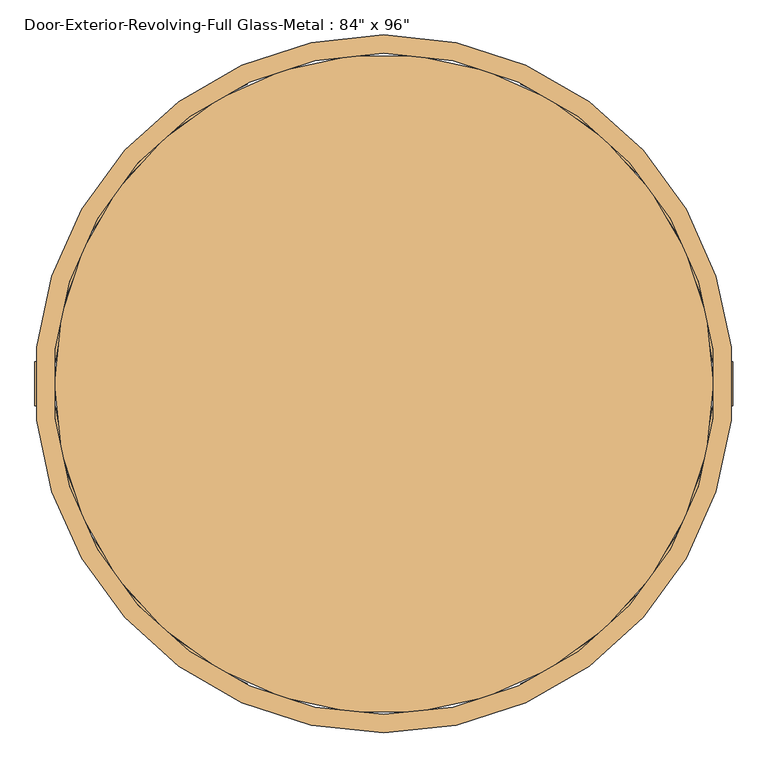
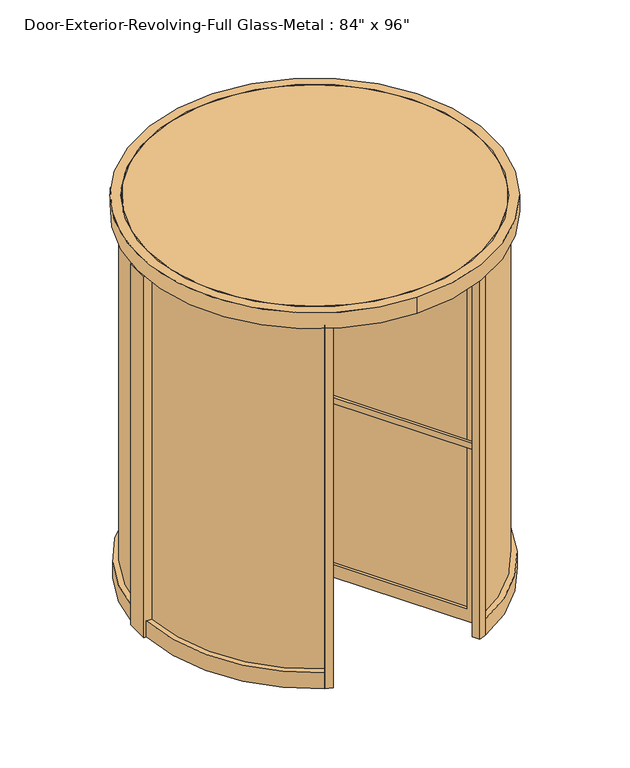
"""IFC4 building model written with IfcOpenShell, lengths in millimetres: door geometry."""

from ifc_helpers import new_model, si_unit, point, frame, frame_2d, origin, origin_with_axes, origin_2d, place, context, project, spatial, polyline, circle_curve, trimmed, segment, composite_curve, outline, extrude, source, transform, mapped, element, save
from ifc_brep_helpers import plane_surface, revolved_surface, advanced_brep


def door_2695eedf(model_context):
    return source(origin(), model_context, "Body", "SolidModel", [
        advanced_brep(
        [(481.9772161, -872.9090263, 25.4), (481.9772161, -872.9090263, 2282.825), (26.9196881, -84.7262674, 2282.825), (26.9196881, -84.7262674, 25.4), (29.5397161, -89.2642891, 2216.15), (448.6397161, -815.1667825, 2216.15), (448.6397161, -815.1667825, 106.3625), (29.5397161, -89.2642891, 106.3625), (514.9727839, -853.8590263, 2282.825), (514.9727839, -853.8590263, 25.4), (59.9152559, -65.6762674, 25.4), (59.9152559, -65.6762674, 2282.825), (62.5352839, -70.2142891, 2216.15), (62.5352839, -70.2142891, 106.3625), (481.6352839, -796.1167825, 106.3625), (481.6352839, -796.1167825, 2216.15), (44.45, -76.9896584, 2282.825), (44.45, -76.9896584, 25.4)],
        [
            (0, 1),
            (1, 2),
            (2, 3),
            (3, 0),
            (4, 5),
            (5, 6),
            (6, 7),
            (7, 4),
            (8, 9),
            (9, 10),
            (10, 11),
            (11, 8),
            (12, 13),
            (13, 14),
            (14, 15),
            (15, 12),
            (1, 8),
            (11, 16, circle_curve(frame((0.0, 0.0, 2282.825), z_axis=(0.0, 0.0, -1.0), x_axis=(0.4999999999999996, -0.8660254037844389, 0.0)), 88.9)),
            (16, 2, circle_curve(frame((0.0, 0.0, 2282.825), z_axis=(0.0, 0.0, -1.0), x_axis=(0.4999999999999996, -0.8660254037844389, 0.0)), 88.9)),
            (0, 9),
            (3, 17, circle_curve(frame((0.0, 0.0, 25.4), z_axis=(0.0, 0.0, 1.0), x_axis=(0.4999999999999996, -0.8660254037844389, 0.0)), 88.9)),
            (17, 10, circle_curve(frame((0.0, 0.0, 25.4), z_axis=(0.0, 0.0, 1.0), x_axis=(0.4999999999999996, -0.8660254037844389, 0.0)), 88.9)),
            (7, 13),
            (12, 4),
            (6, 14),
            (5, 15),
            (16, 17),
        ],
        [
            plane_surface(frame((-3.7977839, -31.5220453, 2282.825), z_axis=(-0.8660254037844389, -0.4999999999999996, 0.0), x_axis=(0.0, 0.0, -1.0))),
            plane_surface(frame((29.1977839, -12.4720453, 2282.825), z_axis=(0.8660254037844389, 0.4999999999999996, 0.0), x_axis=(0.0, 0.0, 1.0))),
            plane_surface(frame((481.9772161, -872.9090263, 2282.825), z_axis=(0.0, 0.0, 1.0), x_axis=(0.8660254037844384, 0.5000000000000004, 0.0))),
            plane_surface(frame((481.9772161, -872.9090263, 25.4), z_axis=(0.5000000000000004, -0.8660254037844384, 0.0), x_axis=(0.8660254037844384, 0.5000000000000004, 0.0))),
            plane_surface(frame((-3.7977839, -31.5220453, 25.4), z_axis=(0.0, 0.0, -1.0), x_axis=(0.8660254037844389, 0.49999999999999956, 0.0))),
            plane_surface(frame((29.5397161, -89.2642891, 106.3625), z_axis=(0.4999999999999998, -0.8660254037844388, 0.0), x_axis=(0.8660254037844388, 0.4999999999999998, 0.0))),
            plane_surface(frame((448.6397161, -815.1667825, 106.3625), z_axis=(0.0, 0.0, 1.0), x_axis=(0.8660254037844384, 0.5000000000000004, 0.0))),
            plane_surface(frame((448.6397161, -815.1667825, 2216.15), z_axis=(-0.5000000000000004, 0.8660254037844384, 0.0), x_axis=(0.8660254037844384, 0.5000000000000004, 0.0))),
            plane_surface(frame((29.5397161, -89.2642891, 2216.15), z_axis=(0.0, 0.0, -1.0), x_axis=(0.8660254037844389, 0.49999999999999967, 0.0))),
            revolved_surface(polyline([(44.44999999999997, -76.98965839643662, 2282.825), (44.44999999999997, -76.98965839643662, 25.399999999999977)]), (0.0, 0.0, -344.4385455), (0.0, 0.0, 1.0)),
        ],
        [
            (0, [[1, 2, 3, 4], [5, 6, 7, 8]]),
            (1, [[9, 10, 11, 12], [13, 14, 15, 16]]),
            (2, [[17, -12, 18, 19, -2]]),
            (3, [[-1, 20, -9, -17]]),
            (4, [[-20, -4, 21, 22, -10]]),
            (5, [[-8, 23, -13, 24]]),
            (6, [[-7, 25, -14, -23]]),
            (7, [[-6, 26, -15, -25]]),
            (8, [[-5, -24, -16, -26]]),
            (9, [[27, -21, -3, -19]]),
            (9, [[-27, -18, -11, -22]]),
        ],
    ),
        advanced_brep(
        [(-996.95, -19.05, 2282.825), (-996.95, -19.05, 25.4), (-86.834944, -19.05, 25.4), (-86.834944, -19.05, 2282.825), (-92.075, -19.05, 2216.15), (-92.075, -19.05, 106.3625), (-930.275, -19.05, 106.3625), (-930.275, -19.05, 2216.15), (-996.95, 19.05, 25.4), (-996.95, 19.05, 2282.825), (-86.834944, 19.05, 2282.825), (-86.834944, 19.05, 25.4), (-92.075, 19.05, 2216.15), (-930.275, 19.05, 2216.15), (-930.275, 19.05, 106.3625), (-92.075, 19.05, 106.3625)],
        [
            (0, 1),
            (1, 2),
            (2, 3),
            (3, 0),
            (4, 5),
            (5, 6),
            (6, 7),
            (7, 4),
            (8, 9),
            (9, 10),
            (10, 11),
            (11, 8),
            (12, 13),
            (13, 14),
            (14, 15),
            (15, 12),
            (9, 0),
            (3, 10, circle_curve(frame((0.0, 0.0, 2282.825), z_axis=(0.0, 0.0, -1.0), x_axis=(0.4999999999999996, -0.8660254037844389, 0.0)), 88.9)),
            (8, 1),
            (11, 2, circle_curve(frame((0.0, 0.0, 25.4), z_axis=(0.0, 0.0, 1.0), x_axis=(0.4999999999999996, -0.8660254037844389, 0.0)), 88.9)),
            (4, 12),
            (15, 5),
            (14, 6),
            (13, 7),
        ],
        [
            plane_surface(frame((-996.95, -19.05, 2282.825), z_axis=(0.0, -1.0, 0.0), x_axis=(-1.0, 0.0, 0.0))),
            plane_surface(frame((-996.95, 19.05, 2282.825), z_axis=(0.0, 1.0, 0.0), x_axis=(1.0, 0.0, 0.0))),
            plane_surface(frame((-25.4, -19.05, 2282.825), z_axis=(0.0, 0.0, 1.0), x_axis=(0.0, 1.0, 0.0))),
            plane_surface(frame((-996.95, -19.05, 2282.825), z_axis=(-1.0, 0.0, 0.0), x_axis=(0.0, 1.0, 0.0))),
            plane_surface(frame((-996.95, -19.05, 25.4), z_axis=(0.0, 0.0, -1.0), x_axis=(0.0, 1.0, 0.0))),
            plane_surface(frame((-92.075, -19.05, 2216.15), z_axis=(-1.0, 0.0, 0.0), x_axis=(0.0, 1.0, 0.0))),
            plane_surface(frame((-92.075, -19.05, 106.3625), z_axis=(0.0, 0.0, 1.0), x_axis=(0.0, 1.0, 0.0))),
            plane_surface(frame((-930.275, -19.05, 106.3625), z_axis=(1.0, 0.0, 0.0), x_axis=(0.0, 1.0, 0.0))),
            plane_surface(frame((-930.275, -19.05, 2216.15), z_axis=(0.0, 0.0, -1.0), x_axis=(0.0, 1.0, 0.0))),
            revolved_surface(polyline([(44.44999999999997, -76.98965839643662, 2282.825), (44.44999999999997, -76.98965839643662, 25.399999999999977)]), (0.0, 0.0, -344.4385455), (0.0, 0.0, 1.0)),
        ],
        [
            (0, [[1, 2, 3, 4], [5, 6, 7, 8]]),
            (1, [[9, 10, 11, 12], [13, 14, 15, 16]]),
            (2, [[17, -4, 18, -10]]),
            (3, [[-1, -17, -9, 19]]),
            (4, [[-19, -12, 20, -2]]),
            (5, [[-5, 21, -16, 22]]),
            (6, [[-6, -22, -15, 23]]),
            (7, [[-7, -23, -14, 24]]),
            (8, [[-8, -24, -13, -21]]),
            (9, [[-3, -20, -11, -18]]),
        ],
    ),
        advanced_brep(
        [(514.9727839, 853.8590263, 25.4), (514.9727839, 853.8590263, 2282.825), (59.9152559, 65.6762674, 2282.825), (59.9152559, 65.6762674, 25.4), (62.5352839, 70.2142891, 2216.15), (481.6352839, 796.1167825, 2216.15), (481.6352839, 796.1167825, 106.3625), (62.5352839, 70.2142891, 106.3625), (481.9772161, 872.9090263, 2282.825), (481.9772161, 872.9090263, 25.4), (26.9196881, 84.7262674, 25.4), (26.9196881, 84.7262674, 2282.825), (29.5397161, 89.2642891, 2216.15), (29.5397161, 89.2642891, 106.3625), (448.6397161, 815.1667825, 106.3625), (448.6397161, 815.1667825, 2216.15)],
        [
            (0, 1),
            (1, 2),
            (2, 3),
            (3, 0),
            (4, 5),
            (5, 6),
            (6, 7),
            (7, 4),
            (8, 9),
            (9, 10),
            (10, 11),
            (11, 8),
            (12, 13),
            (13, 14),
            (14, 15),
            (15, 12),
            (1, 8),
            (11, 2, circle_curve(frame((0.0, 0.0, 2282.825), z_axis=(0.0, 0.0, -1.0), x_axis=(0.4999999999999996, -0.8660254037844389, 0.0)), 88.9)),
            (0, 9),
            (3, 10, circle_curve(frame((0.0, 0.0, 25.4), z_axis=(0.0, 0.0, 1.0), x_axis=(0.4999999999999996, -0.8660254037844389, 0.0)), 88.9)),
            (7, 13),
            (12, 4),
            (6, 14),
            (5, 15),
        ],
        [
            plane_surface(frame((29.1977839, 12.4720453, 2282.825), z_axis=(0.866025403784439, -0.4999999999999995, 0.0), x_axis=(0.0, 0.0, -1.0))),
            plane_surface(frame((-3.7977839, 31.5220453, 2282.825), z_axis=(-0.866025403784439, 0.4999999999999995, 0.0), x_axis=(0.0, 0.0, 1.0))),
            plane_surface(frame((514.9727839, 853.8590263, 2282.825), z_axis=(0.0, 0.0, 1.0), x_axis=(-0.8660254037844384, 0.5000000000000004, 0.0))),
            plane_surface(frame((514.9727839, 853.8590263, 25.4), z_axis=(0.5000000000000004, 0.8660254037844384, 0.0), x_axis=(-0.8660254037844384, 0.5000000000000004, 0.0))),
            plane_surface(frame((29.1977839, 12.4720453, 25.4), z_axis=(0.0, 0.0, -1.0), x_axis=(-0.866025403784439, 0.49999999999999944, 0.0))),
            plane_surface(frame((62.5352839, 70.2142891, 106.3625), z_axis=(0.49999999999999956, 0.8660254037844389, 0.0), x_axis=(-0.8660254037844389, 0.49999999999999956, 0.0))),
            plane_surface(frame((481.6352839, 796.1167825, 106.3625), z_axis=(0.0, 0.0, 1.0), x_axis=(-0.8660254037844384, 0.5000000000000004, 0.0))),
            plane_surface(frame((481.6352839, 796.1167825, 2216.15), z_axis=(-0.5000000000000004, -0.8660254037844384, 0.0), x_axis=(-0.8660254037844384, 0.5000000000000004, 0.0))),
            plane_surface(frame((62.5352839, 70.2142891, 2216.15), z_axis=(0.0, 0.0, -1.0), x_axis=(-0.866025403784439, 0.49999999999999944, 0.0))),
            revolved_surface(polyline([(44.44999999999997, -76.98965839643662, 2282.825), (44.44999999999997, -76.98965839643662, 25.399999999999977)]), (0.0, 0.0, -344.4385455), (0.0, 0.0, 1.0)),
        ],
        [
            (0, [[1, 2, 3, 4], [5, 6, 7, 8]]),
            (1, [[9, 10, 11, 12], [13, 14, 15, 16]]),
            (2, [[17, -12, 18, -2]]),
            (3, [[-1, 19, -9, -17]]),
            (4, [[-19, -4, 20, -10]]),
            (5, [[-8, 21, -13, 22]]),
            (6, [[-7, 23, -14, -21]]),
            (7, [[-6, 24, -15, -23]]),
            (8, [[-5, -22, -16, -24]]),
            (9, [[-3, -18, -11, -20]]),
        ],
    ),
        extrude(outline(composite_curve([segment(polyline([(-463.3921907, 900.6009984), (-485.7275667, 942.9715583)]), True, "CONTINUOUS"), segment(trimmed(circle_curve(origin_2d(), 1060.7198635), [point((-485.7275667, 942.9715583))], [point((-443.2078601, 963.6874086))], False, "CARTESIAN"), True, "CONTINUOUS"), segment(polyline([(-443.2078601, 963.6874086), (-420.8795251, 921.2355323)]), True, "CONTINUOUS"), segment(trimmed(circle_curve(origin_2d(), 1012.825), [point((-420.8795251, 921.2355323))], [point((-463.3921907, 900.6009984))], True, "CARTESIAN"), True, "CONTINUOUS")], self_intersect=False)), origin_with_axes(), (0.0, 0.0, 1.0), 2308.225),
        extrude(outline(composite_curve([segment(polyline([(485.8334006, 943.1723269), (463.3921907, 900.6009984)]), True, "CONTINUOUS"), segment(trimmed(circle_curve(origin_2d(), 1012.825), [point((463.3921907, 900.6009984))], [point((420.8795251, 921.2355323))], True, "CARTESIAN"), True, "CONTINUOUS"), segment(polyline([(420.8795251, 921.2355323), (443.3136707, 963.8885416)]), True, "CONTINUOUS"), segment(trimmed(circle_curve(origin_2d(), 1060.9468089), [point((443.3136707, 963.8885416))], [point((485.8334006, 943.1723269))], False, "CARTESIAN"), True, "CONTINUOUS")], self_intersect=False)), origin_with_axes(), (0.0, 0.0, 1.0), 2308.225),
        extrude(outline(composite_curve([segment(trimmed(circle_curve(origin_2d(), 1012.825), [point((-463.3921907, -900.6009984))], [point((-420.8795251, -921.2355323))], True, "CARTESIAN"), True, "CONTINUOUS"), segment(polyline([(-420.8795251, -921.2355323), (-443.2078601, -959.6749591)]), True, "CONTINUOUS"), segment(trimmed(circle_curve(frame_2d((0.0, 231.0126656)), 1270.4999909), [point((-443.2078601, -959.6749591))], [point((-485.7275667, -942.9715583))], False, "CARTESIAN"), True, "CONTINUOUS"), segment(polyline([(-485.7275667, -942.9715583), (-463.3921907, -900.6009984)]), True, "CONTINUOUS")], self_intersect=False)), origin_with_axes(), (0.0, 0.0, 1.0), 2308.225),
        extrude(outline(composite_curve([segment(trimmed(circle_curve(frame_2d((0.0, 231.0127852)), 1270.5001015), [point((485.7275667, -942.9715583))], [point((443.2078689, -959.6749542))], False, "CARTESIAN"), True, "CONTINUOUS"), segment(polyline([(443.2078689, -959.6749542), (420.8795251, -921.2355323)]), True, "CONTINUOUS"), segment(trimmed(circle_curve(origin_2d(), 1012.825), [point((420.8795251, -921.2355323))], [point((463.3921907, -900.6009984))], True, "CARTESIAN"), True, "CONTINUOUS"), segment(polyline([(463.3921907, -900.6009984), (485.7275667, -942.9715583)]), True, "CONTINUOUS")], self_intersect=False)), origin_with_axes(), (0.0, 0.0, 1.0), 2308.225),
        extrude(outline(composite_curve([segment(polyline([(-1018.5303379, 67.46875), (-1024.8907518, 67.46875)]), True, "CONTINUOUS"), segment(trimmed(circle_curve(origin_2d(), 1027.1090913), [point((-1024.8907518, 67.46875))], [point((-470.5714922, 912.9707312))], False, "CARTESIAN"), True, "CONTINUOUS"), segment(polyline([(-470.5714922, 912.9707312), (-467.3807004, 907.4752681)]), True, "CONTINUOUS"), segment(trimmed(circle_curve(origin_2d(), 1020.7625), [point((-467.3807004, 907.4752681))], [point((-1018.5303379, 67.46875))], True, "CARTESIAN"), True, "CONTINUOUS")], self_intersect=False)), frame((0.0, 0.0, 101.6), z_axis=(0.0, 0.0, 1.0), x_axis=(1.0, 0.0, 0.0)), (0.0, 0.0, 1.0), 2206.625),
        extrude(outline(composite_curve([segment(trimmed(circle_curve(origin_2d(), 1020.7625), [point((1018.5303379, 67.46875))], [point((467.3807004, 907.4752681))], True, "CARTESIAN"), True, "CONTINUOUS"), segment(polyline([(467.3807004, 907.4752681), (470.5714922, 912.9707312)]), True, "CONTINUOUS"), segment(trimmed(circle_curve(origin_2d(), 1027.1090913), [point((470.5714922, 912.9707312))], [point((1024.8907518, 67.46875))], False, "CARTESIAN"), True, "CONTINUOUS"), segment(polyline([(1024.8907518, 67.46875), (1018.5303379, 67.46875)]), True, "CONTINUOUS")], self_intersect=False)), frame((0.0, 0.0, 101.6), z_axis=(0.0, 0.0, 1.0), x_axis=(1.0, 0.0, 0.0)), (0.0, 0.0, 1.0), 2206.625),
        extrude(outline(composite_curve([segment(trimmed(circle_curve(origin_2d(), 1020.7625), [point((-1018.5303379, -67.46875))], [point((-467.3807004, -907.4752681))], True, "CARTESIAN"), True, "CONTINUOUS"), segment(polyline([(-467.3807004, -907.4752681), (-470.5714922, -912.9707312)]), True, "CONTINUOUS"), segment(trimmed(circle_curve(origin_2d(), 1027.1090913), [point((-470.5714922, -912.9707312))], [point((-1024.8907518, -67.46875))], False, "CARTESIAN"), True, "CONTINUOUS"), segment(polyline([(-1024.8907518, -67.46875), (-1018.5303379, -67.46875)]), True, "CONTINUOUS")], self_intersect=False)), frame((0.0, 0.0, 101.6), z_axis=(0.0, 0.0, 1.0), x_axis=(1.0, 0.0, 0.0)), (0.0, 0.0, 1.0), 2206.625),
        extrude(outline(composite_curve([segment(polyline([(1018.5303379, -67.46875), (1024.8907518, -67.46875)]), True, "CONTINUOUS"), segment(trimmed(circle_curve(origin_2d(), 1027.1090913), [point((1024.8907518, -67.46875))], [point((470.5714922, -912.9707312))], False, "CARTESIAN"), True, "CONTINUOUS"), segment(polyline([(470.5714922, -912.9707312), (467.3807004, -907.4752681)]), True, "CONTINUOUS"), segment(trimmed(circle_curve(origin_2d(), 1020.7625), [point((467.3807004, -907.4752681))], [point((1018.5303379, -67.46875))], True, "CARTESIAN"), True, "CONTINUOUS")], self_intersect=False)), frame((0.0, 0.0, 101.6), z_axis=(0.0, 0.0, 1.0), x_axis=(1.0, 0.0, 0.0)), (0.0, 0.0, 1.0), 2206.625),
        extrude(outline(composite_curve([segment(trimmed(circle_curve(origin_2d(), 1073.15), [point((0.0, -1073.15))], [point((0.0, 1073.15))], False, "CARTESIAN"), True, "CONTINUOUS"), segment(trimmed(circle_curve(origin_2d(), 1073.15), [point((0.0, 1073.15))], [point((0.0, -1073.15))], False, "CARTESIAN"), True, "CONTINUOUS")], self_intersect=False), holes=[composite_curve([segment(trimmed(circle_curve(origin_2d(), 1016.0), [point((0.0, 1016.0))], [point((0.0, -1016.0))], True, "CARTESIAN"), True, "CONTINUOUS"), segment(trimmed(circle_curve(origin_2d(), 1016.0), [point((0.0, -1016.0))], [point((0.0, 1016.0))], True, "CARTESIAN"), True, "CONTINUOUS")], self_intersect=False)]), frame((0.0, 0.0, 2308.225), z_axis=(0.0, 0.0, 1.0), x_axis=(1.0, 0.0, 0.0)), (0.0, 0.0, 1.0), 101.6),
        extrude(outline(composite_curve([segment(trimmed(circle_curve(origin_2d(), 1012.825), [point((-1012.825, 0.0))], [point((1012.825, 0.0))], False, "CARTESIAN"), True, "CONTINUOUS"), segment(trimmed(circle_curve(origin_2d(), 1012.825), [point((1012.825, 0.0))], [point((-1012.825, 0.0))], False, "CARTESIAN"), True, "CONTINUOUS")], self_intersect=False)), frame((0.0, 0.0, 2308.225), z_axis=(0.0, 0.0, 1.0), x_axis=(1.0, 0.0, 0.0)), (0.0, 0.0, 1.0), 101.6),
        extrude(outline(composite_curve([segment(trimmed(circle_curve(origin_2d(), 88.9), [point((-88.9, 0.0))], [point((88.9, 0.0))], False, "CARTESIAN"), True, "CONTINUOUS"), segment(trimmed(circle_curve(origin_2d(), 88.9), [point((88.9, 0.0))], [point((-88.9, 0.0))], False, "CARTESIAN"), True, "CONTINUOUS")], self_intersect=False)), origin_with_axes(), (0.0, 0.0, 1.0), 2308.225),
        extrude(outline(composite_curve([segment(polyline([(-463.3921907, -900.6009984), (-485.7275667, -942.9715583)]), True, "CONTINUOUS"), segment(trimmed(circle_curve(origin_2d(), 1060.7198635), [point((-485.7275667, -942.9715583))], [point((-1058.571961, -67.46875))], False, "CARTESIAN"), True, "CONTINUOUS"), segment(polyline([(-1058.571961, -67.46875), (-1010.5753057, -67.46875)]), True, "CONTINUOUS"), segment(trimmed(circle_curve(origin_2d(), 1012.825), [point((-1010.5753057, -67.46875))], [point((-463.3921907, -900.6009984))], True, "CARTESIAN"), True, "CONTINUOUS")], self_intersect=False)), origin_with_axes(), (0.0, 0.0, 1.0), 101.6),
        extrude(outline(composite_curve([segment(polyline([(485.7275667, -942.9715583), (463.3921907, -900.6009984)]), True, "CONTINUOUS"), segment(trimmed(circle_curve(origin_2d(), 1012.825), [point((463.3921907, -900.6009984))], [point((1010.5753057, -67.46875))], True, "CARTESIAN"), True, "CONTINUOUS"), segment(polyline([(1010.5753057, -67.46875), (1058.571961, -67.46875)]), True, "CONTINUOUS"), segment(trimmed(circle_curve(origin_2d(), 1060.7198635), [point((1058.571961, -67.46875))], [point((485.7275667, -942.9715583))], False, "CARTESIAN"), True, "CONTINUOUS")], self_intersect=False)), origin_with_axes(), (0.0, 0.0, 1.0), 101.6),
        extrude(outline(composite_curve([segment(polyline([(1058.571961, 67.46875), (1010.5753057, 67.46875)]), True, "CONTINUOUS"), segment(trimmed(circle_curve(origin_2d(), 1012.825), [point((1010.5753057, 67.46875))], [point((463.3921907, 900.6009984))], True, "CARTESIAN"), True, "CONTINUOUS"), segment(polyline([(463.3921907, 900.6009984), (485.7275667, 942.9715583)]), True, "CONTINUOUS"), segment(trimmed(circle_curve(origin_2d(), 1060.7198635), [point((485.7275667, 942.9715583))], [point((1058.571961, 67.46875))], False, "CARTESIAN"), True, "CONTINUOUS")], self_intersect=False)), origin_with_axes(), (0.0, 0.0, 1.0), 101.6),
        extrude(outline(composite_curve([segment(polyline([(-485.7275667, 942.9715583), (-463.3921907, 900.6009984)]), True, "CONTINUOUS"), segment(trimmed(circle_curve(origin_2d(), 1012.825), [point((-463.3921907, 900.6009984))], [point((-1010.5753057, 67.46875))], True, "CARTESIAN"), True, "CONTINUOUS"), segment(polyline([(-1010.5753057, 67.46875), (-1058.571961, 67.46875)]), True, "CONTINUOUS"), segment(trimmed(circle_curve(origin_2d(), 1060.7198635), [point((-1058.571961, 67.46875))], [point((-485.7275667, 942.9715583))], False, "CARTESIAN"), True, "CONTINUOUS")], self_intersect=False)), origin_with_axes(), (0.0, 0.0, 1.0), 101.6),
        extrude(outline(polyline([(-1016.0, 67.46875), (-1016.0, -67.46875), (-1073.15, -67.46875), (-1073.15, 67.46875), (-1016.0, 67.46875)])), origin_with_axes(), (0.0, 0.0, 1.0), 2308.225),
        extrude(outline(polyline([(1073.15, 67.46875), (1073.15, -67.46875), (1016.0, -67.46875), (1016.0, 67.46875), (1073.15, 67.46875)])), origin_with_axes(), (0.0, 0.0, 1.0), 2308.225),
        extrude(outline(polyline([(462.3878693, -807.2292825), (43.2878693, -81.3267891), (48.7871307, -78.1517891), (467.8871307, -804.0542825), (462.3878693, -807.2292825)])), frame((0.0, 0.0, 106.3625), z_axis=(0.0, 0.0, 1.0), x_axis=(1.0, 0.0, 0.0)), (0.0, 0.0, 1.0), 2109.7875),
        extrude(outline(polyline([(467.8871307, 804.0542825), (48.7871307, 78.1517891), (43.2878693, 81.3267891), (462.3878693, 807.2292825), (467.8871307, 804.0542825)])), frame((0.0, 0.0, 106.3625), z_axis=(0.0, 0.0, 1.0), x_axis=(1.0, 0.0, 0.0)), (0.0, 0.0, 1.0), 2109.7875),
        extrude(outline(polyline([(-92.075, -3.175), (-930.275, -3.175), (-930.275, 3.175), (-92.075, 3.175), (-92.075, -3.175)])), frame((0.0, 0.0, 106.3625), z_axis=(0.0, 0.0, 1.0), x_axis=(1.0, 0.0, 0.0)), (0.0, 0.0, 1.0), 2109.7875),
        extrude(outline(composite_curve([segment(polyline([(-996.95, 19.05), (-996.95, 38.1), (-80.3218526, 38.1)]), True, "CONTINUOUS"), segment(trimmed(circle_curve(origin_2d(), 88.9), [point((-80.3218526, 38.1))], [point((-86.834944, 19.05))], True, "CARTESIAN"), True, "CONTINUOUS"), segment(polyline([(-86.834944, 19.05), (-996.95, 19.05)]), True, "CONTINUOUS")], self_intersect=False)), frame((0.0, 0.0, 1149.35), z_axis=(0.0, 0.0, 1.0), x_axis=(1.0, 0.0, 0.0)), (0.0, 0.0, 1.0), 38.1),
        extrude(outline(composite_curve([segment(polyline([(481.9772161, -872.9090263), (465.4794321, -882.4340263), (7.1653584, -88.6107648)]), True, "CONTINUOUS"), segment(trimmed(circle_curve(origin_2d(), 88.9), [point((7.1653584, -88.6107648))], [point((26.9196881, -84.7262674))], True, "CARTESIAN"), True, "CONTINUOUS"), segment(polyline([(26.9196881, -84.7262674), (481.9772161, -872.9090263)]), True, "CONTINUOUS")], self_intersect=False)), frame((0.0, 0.0, 1149.35), z_axis=(0.0, 0.0, 1.0), x_axis=(1.0, 0.0, 0.0)), (0.0, 0.0, 1.0), 38.1),
        extrude(outline(composite_curve([segment(polyline([(514.9727839, 853.8590263), (531.4705679, 844.3340263), (73.1564942, 50.5107648)]), True, "CONTINUOUS"), segment(trimmed(circle_curve(origin_2d(), 88.9), [point((73.1564942, 50.5107648))], [point((59.9152559, 65.6762674))], True, "CARTESIAN"), True, "CONTINUOUS"), segment(polyline([(59.9152559, 65.6762674), (514.9727839, 853.8590263)]), True, "CONTINUOUS")], self_intersect=False)), frame((0.0, 0.0, 1149.35), z_axis=(0.0, 0.0, 1.0), x_axis=(1.0, 0.0, 0.0)), (0.0, 0.0, 1.0), 38.1),
    ])


if __name__ == "__main__":
    model = new_model("IFC4")
    model_context = context("Model", 3, world=origin())
    ifc_project = project(units=[si_unit("LENGTHUNIT", "METRE", prefix="MILLI")], contexts=[model_context])
    site = spatial("IfcSite", under=ifc_project)
    building = spatial("IfcBuilding", under=site)
    placement = place(None, origin())
    door_shape = door_2695eedf(model_context)
    element("IfcDoor", 1, ObjectType="Door-Exterior-Revolving-Full Glass-Metal : 84\" x 96\"", at=placement, inside=building, context=model_context, shape_type="MappedRepresentation", body=[
        mapped(door_shape, transform((0.0, 0.0, 0.0), x_axis=(1.0, 0.0, 0.0), y_axis=(0.0, 1.0, 0.0), z_axis=(0.0, 0.0, 1.0))),
    ])
    save(model, "model.ifc")

# Revit data of these elements
# Type "Door-Exterior-Revolving-Full Glass-Metal : 84\" x 96\""
#   Type Mark = "19"
#   Assembly Code = "B2030100"
#   Analytic Construction = "Metal frame, double glass door"
#   Panel Width = 3' - 2 1/4"
#   Thermal Resistance (R) = 1.3794 (h·ft²·°F)/BTU
#   Rough Width = 7' - 0 1/2"
#   Rough Height = 7' - 10 7/8"
#   Outside Diameter = 7' - 0 1/2"
#   Push Bar Height = 3' - 10"
#   Inside Radius = 3' - 3 7/8"
#   Inside Diameter = 6' - 7 3/4"
#   Heat Transfer Coefficient (U) = 0.7250 BTU/(h·ft²·°F)
#   Glazing Radius = 3' - 4 3/16"
#   Height = 7' - 10 1/2"
#   Width = 7' - 0"
#   Door Opening Width = 2' - 9 1/8"
#   Function = 1
#   Push Bar Material = Aluminum
#   Panel Material = Aluminum
#   Glazing = Glass
#   Frame Material = Aluminum
#   Visual Light Transmittance = 0
#   Solar Heat Gain Coefficient = 0
#   Wall Closure = (empty or 0)
# Element 1 (IfcDoor, "Door-Exterior-Revolving-Full Glass-Metal : 84\" x 96\"")
#   Materials on its faces: "Aluminum", "Glass"
# Materials
#   "Aluminum": class "Metal", colour RGB 247 247 247, transparency 0, Description = "Aluminum 6061", Cost = 0
#   "Glass": class "Glass", colour RGB 0 128 192, transparency 0.75, Description = "Soda Lime Glass", Cost = 0
